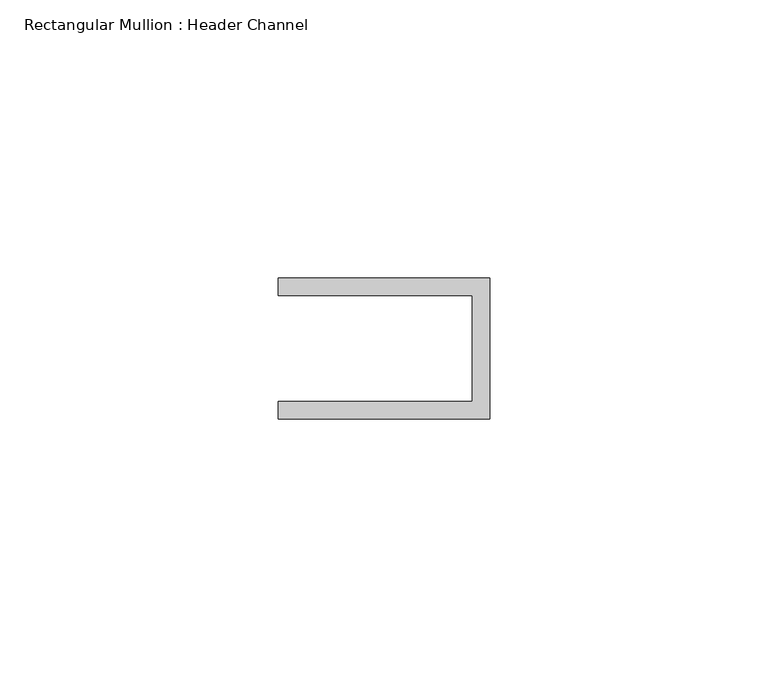
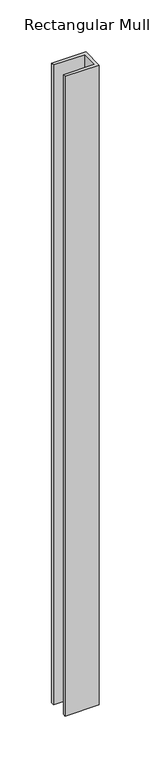
"""IFC4 building model written with IfcOpenShell, lengths in millimetres: member geometry, Rectangular Mullion : Header Channel."""

from ifc_helpers import new_model, si_unit, frame, origin, place, context, project, spatial, polyline, outline, extrude, source, transform, mapped, element, save


def rectangular_mullion_header_channel_76e8dcff(model_context):
    return source(origin(), model_context, "Body", "SweptSolid", [
        extrude(outline(polyline([(0.0, -12.7), (-38.1, -12.7), (-38.1, -9.525), (-3.175, -9.525), (-3.175, 9.525), (-38.1, 9.525), (-38.1, 12.7), (0.0, 12.7), (0.0, -12.7)])), frame((0.0, 0.0, -751.4166667), z_axis=(0.0, 0.0, 1.0), x_axis=(1.0, 0.0, 0.0)), (0.0, 0.0, 1.0), 751.4166667),
    ])


if __name__ == "__main__":
    model = new_model("IFC4")
    model_context = context("Model", 3, world=origin())
    ifc_project = project(units=[si_unit("LENGTHUNIT", "METRE", prefix="MILLI")], contexts=[model_context])
    site = spatial("IfcSite", under=ifc_project)
    building = spatial("IfcBuilding", under=site)
    placement = place(None, origin())
    rectangular_mullion_header_channel_shape = rectangular_mullion_header_channel_76e8dcff(model_context)
    element("IfcMember", 1, ObjectType="Rectangular Mullion : Header Channel", at=placement, inside=building, context=model_context, shape_type="MappedRepresentation", body=[
        mapped(rectangular_mullion_header_channel_shape, transform((0.0, 0.0, 0.0), x_axis=(1.0, 0.0, 0.0), y_axis=(0.0, 1.0, 0.0), z_axis=(0.0, 0.0, 1.0))),
    ])
    save(model, "model.ifc")

# Revit data of these elements
# Type "Rectangular Mullion : Header Channel"
#   built-in parameter 1007322 = 0.0833333 (stored number, unit not read)
#   built-in parameter 1007321 = -0.03125 (stored number, unit not read)
#   built-in parameter 1007320 = 0.0416667 (stored number, unit not read)
# Element 1 (IfcMember, "Rectangular Mullion : Header Channel")
#   Materials on its faces: "ALUM"
# Materials
#   "ALUM": class "Generic", colour RGB 157 157 157, transparency 0, Cost = 0
